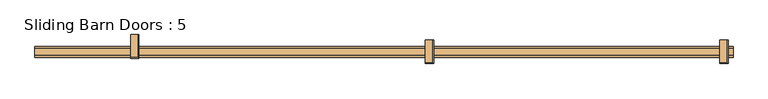
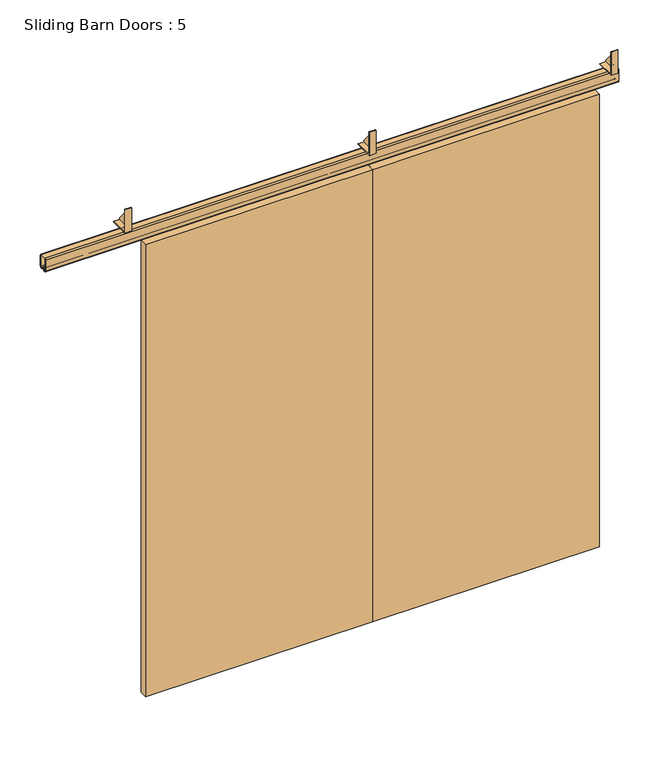
"""IFC4 building model written with IfcOpenShell, lengths in millimetres: door geometry, Sliding Barn Doors : 5."""

import ifcopenshell
import ifcopenshell.guid

model = None  # the IFC model being written
_history = None  # IfcOwnerHistory: only IFC2X3 demands one
_inside = {}  # id of a spatial element -> (the spatial element, [elements in it])
_under = {}  # id of a project, library or spatial element -> (it, [spatial elements below it])
_declared = {}  # id of a project -> (the project, [libraries it declares])
_typed = {}  # id of a type object -> (the type object, [elements of that type])
_made_of = {}  # id of a material, layer set ... -> (it, [elements and type objects made of it])


def new_model(schema):
    """Start an empty IFC model of exactly this schema.

    Asked for "IFC4X3", IfcOpenShell would pick the latest addendum, in which some entities
    have other attributes; the version numbers below select the first issue.
    IFC2X3 requires an IfcOwnerHistory on every rooted entity: one is made here for all.
    """
    global model, _history
    if schema == "IFC4X3":
        model = ifcopenshell.file(schema_version=(4, 3, 0, 0))
    else:
        model = ifcopenshell.file(schema=schema)
    _inside.clear()
    _under.clear()
    _declared.clear()
    _typed.clear()
    _made_of.clear()
    _history = None
    if model.schema == "IFC2X3":
        org = make("IfcOrganization", Name="unknown")
        user = make(
            "IfcPersonAndOrganization",
            ThePerson=make("IfcPerson", FamilyName="unknown"),
            TheOrganization=org,
        )
        app = make(
            "IfcApplication",
            ApplicationDeveloper=org,
            Version="unknown",
            ApplicationFullName="unknown",
            ApplicationIdentifier="unknown",
        )
        _history = make(
            "IfcOwnerHistory",
            OwningUser=user,
            OwningApplication=app,
            ChangeAction="ADDED",
            CreationDate=0,
        )
    return model


def make(cls, **values):
    """One entity of the class cls with the attributes given. An attribute that is None is left unset."""
    return model.create_entity(
        cls, **{name: value for name, value in values.items() if value is not None}
    )


def rooted(cls, **values):
    """An entity with a GlobalId (a new one), such as an element, a storey or a relation."""
    return make(cls, GlobalId=ifcopenshell.guid.new(), OwnerHistory=_history, **values)


def si_unit(unit_type, name, prefix=None):
    """IfcSIUnit, for example si_unit("LENGTHUNIT", "METRE", prefix="MILLI")."""
    return make("IfcSIUnit", UnitType=unit_type, Prefix=prefix, Name=name)


def assignment(units):
    """IfcUnitAssignment: the units of a project."""
    return None if units is None else make("IfcUnitAssignment", Units=units)


def point(xyz):
    """IfcCartesianPoint."""
    return None if xyz is None else make("IfcCartesianPoint", Coordinates=xyz)


def direction(xyz):
    """IfcDirection."""
    return None if xyz is None else make("IfcDirection", DirectionRatios=xyz)


def frame(location, z_axis=None, x_axis=None):
    """IfcAxis2Placement3D, a coordinate frame: its origin and axes. An axis left out is left unset."""
    return make(
        "IfcAxis2Placement3D",
        Location=point(location),
        Axis=direction(z_axis),
        RefDirection=direction(x_axis),
    )


def frame_2d(location, x_axis=None):
    """IfcAxis2Placement2D, a coordinate frame in the plane: its origin and x axis."""
    return make(
        "IfcAxis2Placement2D", Location=point(location), RefDirection=direction(x_axis)
    )


def origin():
    """The frame at (0, 0, 0) with its axes left unset."""
    return frame((0.0, 0.0, 0.0))


def place(relative_to, where):
    """IfcLocalPlacement: puts the frame where relative to a parent placement (None: the world)."""
    return make(
        "IfcLocalPlacement", PlacementRelTo=relative_to, RelativePlacement=where
    )


def context(
    kind, dimensions, precision=None, world=None, true_north=None, identifier=None
):
    """IfcGeometricRepresentationContext, for example the 3D "Model" context."""
    return make(
        "IfcGeometricRepresentationContext",
        ContextIdentifier=identifier,
        ContextType=kind,
        CoordinateSpaceDimension=dimensions,
        Precision=precision,
        WorldCoordinateSystem=world,
        TrueNorth=true_north,
    )


def project(units=None, contexts=None):
    """IfcProject with its units and contexts."""
    return rooted(
        "IfcProject",
        Name="project",
        RepresentationContexts=contexts,
        UnitsInContext=assignment(units),
    )


def spatial(cls, under=None, at=None, **own):
    """A site, building, storey or space (cls), placed at a placement, below another one or the project."""
    s = rooted(cls, ObjectPlacement=at, **own)
    if under is not None:
        _under.setdefault(under.id(), (under, []))[1].append(s)
    return s


def polyline(points):
    """IfcPolyline through the points."""
    return make("IfcPolyline", Points=[point(p) for p in points])


def circle_curve(where, radius):
    """IfcCircle in the frame where."""
    return make("IfcCircle", Position=where, Radius=radius)


def trimmed(basis, trim1, trim2, sense, master):
    """IfcTrimmedCurve: the piece of a basis curve between two trims."""
    return make(
        "IfcTrimmedCurve",
        BasisCurve=basis,
        Trim1=trim1,
        Trim2=trim2,
        SenseAgreement=sense,
        MasterRepresentation=master,
    )


def segment(curve, same_sense, transition):
    """IfcCompositeCurveSegment."""
    return make(
        "IfcCompositeCurveSegment",
        Transition=transition,
        SameSense=same_sense,
        ParentCurve=curve,
    )


def composite_curve(segments, self_intersect=None):
    """IfcCompositeCurve: segments joined end to end."""
    return make("IfcCompositeCurve", Segments=segments, SelfIntersect=self_intersect)


def outline(outer, holes=None, kind="AREA"):
    """IfcArbitraryClosedProfileDef: a profile drawn as a closed curve; with holes, ...WithVoids."""
    if holes is None:
        return make("IfcArbitraryClosedProfileDef", ProfileType=kind, OuterCurve=outer)
    return make(
        "IfcArbitraryProfileDefWithVoids",
        ProfileType=kind,
        OuterCurve=outer,
        InnerCurves=holes,
    )


def extrude(swept, where, along, depth):
    """IfcExtrudedAreaSolid: the profile swept, set in the frame where, extruded along a direction by depth."""
    return make(
        "IfcExtrudedAreaSolid",
        SweptArea=swept,
        Position=where,
        ExtrudedDirection=direction(along),
        Depth=depth,
    )


def shape(context_of_items, identifier, shape_type, items):
    """IfcShapeRepresentation: the items that make up one representation, for example the "Body"."""
    return make(
        "IfcShapeRepresentation",
        ContextOfItems=context_of_items,
        RepresentationIdentifier=identifier,
        RepresentationType=shape_type,
        Items=items,
    )


def source(mapping_origin, context_of_items, identifier, shape_type, items):
    """IfcRepresentationMap: a shape defined once, which mapped items show again and again."""
    return make(
        "IfcRepresentationMap",
        MappingOrigin=mapping_origin,
        MappedRepresentation=shape(context_of_items, identifier, shape_type, items),
    )


def transform(
    local_origin,
    x_axis=None,
    y_axis=None,
    z_axis=None,
    scale=None,
    scale2=None,
    scale3=None,
    uniform=True,
):
    """IfcCartesianTransformationOperator3D, or its non-uniform kind. x_axis, y_axis, z_axis: its Axis1, 2, 3."""
    if uniform:
        return make(
            "IfcCartesianTransformationOperator3D",
            Axis1=direction(x_axis),
            Axis2=direction(y_axis),
            LocalOrigin=point(local_origin),
            Scale=scale,
            Axis3=direction(z_axis),
        )
    return make(
        "IfcCartesianTransformationOperator3DnonUniform",
        Axis1=direction(x_axis),
        Axis2=direction(y_axis),
        LocalOrigin=point(local_origin),
        Scale=scale,
        Axis3=direction(z_axis),
        Scale2=scale2,
        Scale3=scale3,
    )


def mapped(mapping_source, mapping_target):
    """IfcMappedItem: shows the shape of a source again, moved by a transform."""
    return make(
        "IfcMappedItem", MappingSource=mapping_source, MappingTarget=mapping_target
    )


def made_of(thing, what):
    """Note that an element or type object is made of a material, layer set ...; save() writes the relation."""
    if what is not None:
        _made_of.setdefault(what.id(), (what, []))[1].append(thing)
    return thing


def element(
    cls,
    number,
    at=None,
    inside=None,
    cuts=None,
    type_object=None,
    material=None,
    context=None,
    identifier="Body",
    shape_type=None,
    held_by="IfcProductDefinitionShape",
    body=None,
    shapes=None,
    **own,
):
    """One element of the class cls, such as IfcWall. Its Tag is "e" and its number.

    at: its placement. inside: the storey or other place that contains it. cuts: it is an
    opening in that element (IfcRelVoidsElement). A single representation is given by context,
    identifier, shape_type and body (its items); several are given by shapes. held_by: the class
    of the entity that holds the representations. save() writes the other relations.
    """
    e = rooted(cls, Tag="e%d" % number, ObjectPlacement=at, **own)
    if body is not None:
        shapes = [shape(context, identifier, shape_type, body)]
    if shapes is not None:
        e.Representation = make(held_by, Representations=shapes)
    if inside is not None:
        _inside.setdefault(inside.id(), (inside, []))[1].append(e)
    if cuts is not None:
        rooted(
            "IfcRelVoidsElement", RelatingBuildingElement=cuts, RelatedOpeningElement=e
        )
    if type_object is not None:
        _typed.setdefault(type_object.id(), (type_object, []))[1].append(e)
    return made_of(e, material)


def aggregate(whole, parts):
    """IfcRelAggregates: a whole, such as a stair, and the parts it consists of."""
    return rooted("IfcRelAggregates", RelatingObject=whole, RelatedObjects=parts)


def save(model, path):
    """Write the relations noted so far, then the file.

    IfcRelAggregates (storeys below a building ...), IfcRelContainedInSpatialStructure (elements
    in a storey), IfcRelDefinesByType, IfcRelAssociatesMaterial and IfcRelDeclares: one each for
    every whole, place, type object, material and project.
    """
    for whole, parts in _under.values():
        aggregate(whole, parts)
    for where, things in _inside.values():
        rooted(
            "IfcRelContainedInSpatialStructure",
            RelatedElements=things,
            RelatingStructure=where,
        )
    for kind, things in _typed.values():
        rooted("IfcRelDefinesByType", RelatedObjects=things, RelatingType=kind)
    for what, things in _made_of.values():
        rooted("IfcRelAssociatesMaterial", RelatedObjects=things, RelatingMaterial=what)
    for by, libraries in _declared.values():
        rooted("IfcRelDeclares", RelatingContext=by, RelatedDefinitions=libraries)
    model.write(path)


def sliding_barn_doors_5_db2e6e72(model_context):
    return source(origin(), model_context, "Body", "SweptSolid", [
        extrude(outline(polyline([(158.75, 2152.65), (158.75, 2146.3), (79.375, 2146.3), (79.375, 2247.773), (158.75, 2152.65)])), frame((-1512.9371094, 0.0, 0.0), z_axis=(1.0, 0.0, 0.0), x_axis=(0.0, 1.0, 0.0)), (0.0, 0.0, 1.0), 3.175),
        extrude(outline(polyline([(76.2, 2143.125), (76.2, 2247.773), (79.375, 2247.773), (79.375, 2146.3), (158.75, 2146.3), (158.75, 2143.125), (76.2, 2143.125)])), frame((-1538.2378906, 0.0, 0.0), z_axis=(1.0, 0.0, 0.0), x_axis=(0.0, 1.0, 0.0)), (0.0, 0.0, 1.0), 28.4757812),
        extrude(outline(polyline([(139.7, 2152.65), (139.7, 2146.3), (60.325, 2146.3), (60.325, 2247.773), (139.7, 2152.65)])), frame((-484.2371094, 0.0, 0.0), z_axis=(1.0, 0.0, 0.0), x_axis=(0.0, 1.0, 0.0)), (0.0, 0.0, 1.0), 3.175),
        extrude(outline(polyline([(57.15, 2143.125), (57.15, 2247.773), (60.325, 2247.773), (60.325, 2146.3), (139.7, 2146.3), (139.7, 2143.125), (57.15, 2143.125)])), frame((-509.5378906, 0.0, 0.0), z_axis=(1.0, 0.0, 0.0), x_axis=(0.0, 1.0, 0.0)), (0.0, 0.0, 1.0), 28.4757813),
        extrude(outline(polyline([(139.7, 2152.65), (139.7, 2146.3), (60.325, 2146.3), (60.325, 2247.773), (139.7, 2152.65)])), frame((544.4628906, 0.0, 0.0), z_axis=(1.0, 0.0, 0.0), x_axis=(0.0, 1.0, 0.0)), (0.0, 0.0, 1.0), 3.175),
        extrude(outline(polyline([(57.15, 2143.125), (57.15, 2247.773), (60.325, 2247.773), (60.325, 2146.3), (139.7, 2146.3), (139.7, 2143.125), (57.15, 2143.125)])), frame((519.1621094, 0.0, 0.0), z_axis=(1.0, 0.0, 0.0), x_axis=(0.0, 1.0, 0.0)), (0.0, 0.0, 1.0), 28.4757813),
        extrude(outline(polyline([(-1346.454, 117.475), (-1295.146, 117.475), (-1295.146, 114.3), (-1346.454, 114.3), (-1346.454, 117.475)])), frame((0.0, 0.0, 1889.252), z_axis=(0.0, 0.0, 1.0), x_axis=(1.0, 0.0, 0.0)), (0.0, 0.0, 1.0), 168.148),
        extrude(outline(polyline([(-635.254, 117.475), (-583.946, 117.475), (-583.946, 114.3), (-635.254, 114.3), (-635.254, 117.475)])), frame((0.0, 0.0, 1889.252), z_axis=(0.0, 0.0, 1.0), x_axis=(1.0, 0.0, 0.0)), (0.0, 0.0, 1.0), 168.148),
        extrude(outline(polyline([(-381.254, 117.475), (-329.946, 117.475), (-329.946, 114.3), (-381.254, 114.3), (-381.254, 117.475)])), frame((0.0, 0.0, 1889.252), z_axis=(0.0, 0.0, 1.0), x_axis=(1.0, 0.0, 0.0)), (0.0, 0.0, 1.0), 168.148),
        extrude(outline(polyline([(329.946, 117.475), (381.254, 117.475), (381.254, 114.3), (329.946, 114.3), (329.946, 117.475)])), frame((0.0, 0.0, 1889.252), z_axis=(0.0, 0.0, 1.0), x_axis=(1.0, 0.0, 0.0)), (0.0, 0.0, 1.0), 168.148),
        extrude(outline(polyline([(-1447.8, 114.3), (-482.6, 114.3), (-482.6, 79.375), (-1447.8, 79.375), (-1447.8, 114.3)])), frame((0.0, 0.0, 25.4), z_axis=(0.0, 0.0, 1.0), x_axis=(1.0, 0.0, 0.0)), (0.0, 0.0, 1.0), 2032.0),
        extrude(outline(polyline([(-482.6, 114.3), (482.6, 114.3), (482.6, 79.375), (-482.6, 79.375), (-482.6, 114.3)])), frame((0.0, 0.0, 25.4), z_axis=(0.0, 0.0, 1.0), x_axis=(1.0, 0.0, 0.0)), (0.0, 0.0, 1.0), 2032.0),
        extrude(outline(composite_curve([segment(polyline([(85.725, 2143.125), (111.252, 2143.125)]), True, "CONTINUOUS"), segment(trimmed(circle_curve(frame_2d((111.252, 2136.775)), 6.35), [point((111.252, 2143.125))], [point((117.602, 2136.775))], False, "CARTESIAN"), True, "CONTINUOUS"), segment(polyline([(117.602, 2136.775), (117.602, 2088.515)]), True, "CONTINUOUS"), segment(trimmed(circle_curve(frame_2d((111.252, 2088.515)), 6.35), [point((117.602, 2088.515))], [point((111.252, 2082.165))], False, "CARTESIAN"), True, "CONTINUOUS"), segment(polyline([(111.252, 2082.165), (105.8433147, 2082.165)]), True, "CONTINUOUS"), segment(trimmed(circle_curve(frame_2d((105.8433147, 2083.7525)), 1.5875), [point((105.8433147, 2082.165))], [point((104.2849816, 2083.4495907))], False, "CARTESIAN"), True, "CONTINUOUS"), segment(polyline([(104.2849816, 2083.4495907), (102.8594659, 2090.7832331), (104.3756029, 2090.7832331), (105.7615251, 2083.6532812), (111.252, 2083.6532812)]), True, "CONTINUOUS"), segment(trimmed(circle_curve(frame_2d((111.252, 2088.515)), 4.8617187), [point((111.252, 2083.6532812))], [point((116.1137188, 2088.515))], True, "CARTESIAN"), True, "CONTINUOUS"), segment(polyline([(116.1137188, 2088.515), (116.1137188, 2136.775)]), True, "CONTINUOUS"), segment(trimmed(circle_curve(frame_2d((111.252, 2136.775)), 4.8617187), [point((116.1137188, 2136.775))], [point((111.252, 2141.6367187))], True, "CARTESIAN"), True, "CONTINUOUS"), segment(polyline([(111.252, 2141.6367187), (85.725, 2141.6367187)]), True, "CONTINUOUS"), segment(trimmed(circle_curve(frame_2d((85.725, 2136.775)), 4.8617187), [point((85.725, 2141.6367187))], [point((80.8632813, 2136.775))], True, "CARTESIAN"), True, "CONTINUOUS"), segment(polyline([(80.8632813, 2136.775), (80.8632813, 2088.515)]), True, "CONTINUOUS"), segment(trimmed(circle_curve(frame_2d((85.725, 2088.515)), 4.8617187), [point((80.8632813, 2088.515))], [point((85.725, 2083.6532812))], True, "CARTESIAN"), True, "CONTINUOUS"), segment(polyline([(85.725, 2083.6532812), (91.2154749, 2083.6532812), (92.6013971, 2090.7832331), (94.1175341, 2090.7832331), (92.6920184, 2083.4495907)]), True, "CONTINUOUS"), segment(trimmed(circle_curve(frame_2d((91.1336853, 2083.7525)), 1.5875), [point((92.6920184, 2083.4495907))], [point((91.1336853, 2082.165))], False, "CARTESIAN"), True, "CONTINUOUS"), segment(polyline([(91.1336853, 2082.165), (85.725, 2082.165)]), True, "CONTINUOUS"), segment(trimmed(circle_curve(frame_2d((85.725, 2088.515)), 6.35), [point((85.725, 2082.165))], [point((79.375, 2088.515))], False, "CARTESIAN"), True, "CONTINUOUS"), segment(polyline([(79.375, 2088.515), (79.375, 2136.775)]), True, "CONTINUOUS"), segment(trimmed(circle_curve(frame_2d((85.725, 2136.775)), 6.35), [point((79.375, 2136.775))], [point((85.725, 2143.125))], False, "CARTESIAN"), True, "CONTINUOUS")], self_intersect=False)), frame((-1873.25, 0.0, 0.0), z_axis=(1.0, 0.0, 0.0), x_axis=(0.0, 1.0, 0.0)), (0.0, 0.0, 1.0), 2438.4),
    ])


if __name__ == "__main__":
    model = new_model("IFC4")
    model_context = context("Model", 3, world=origin())
    ifc_project = project(units=[si_unit("LENGTHUNIT", "METRE", prefix="MILLI")], contexts=[model_context])
    site = spatial("IfcSite", under=ifc_project)
    building = spatial("IfcBuilding", under=site)
    placement = place(None, origin())
    sliding_barn_doors_5_shape = sliding_barn_doors_5_db2e6e72(model_context)
    element("IfcDoor", 1, ObjectType="Sliding Barn Doors : 5", at=placement, inside=building, context=model_context, shape_type="MappedRepresentation", body=[
        mapped(sliding_barn_doors_5_shape, transform((0.0, 0.0, 0.0), x_axis=(1.0, 0.0, 0.0), y_axis=(0.0, 1.0, 0.0), z_axis=(0.0, 0.0, 1.0))),
    ])
    save(model, "model.ifc")

# Revit data of these elements
# Type "Sliding Barn Doors : 5"
#   Type Mark = "46"
#   Analytic Construction = "<None>"
#   rail_overlap_left = 0' - 5 1/4"
#   rail_length = 8' - 0"
#   overlap_left = 0' - 2"
#   overlap = 0' - 0"
#   bracket_right = 3' - 7"
#   bracket_left = 0' - 4"
#   Thickness = 0' - 1 3/8"
#   Panel Width = 3' - 2"
#   Panel Height = 6' - 8"
#   Gap 2 = 0' - 0 1/2"
#   Gap 1 = 0' - 0 7/8"
#   Frame Projection Ext. = 0' - 1"
#   Frame Projection Int. = 0' - 1"
#   Frame Width = 0' - 3"
#   Height = 6' - 4"
#   Width = 2' - 10"
#   Bracket_offset = 0' - 5"
#   Door_4 = no
#   Door_3 = no
#   Hardware Material = Metal - Aluminum
#   Door Material = Closet_1
#   Function = (empty or 0)
#   Wall Closure = (empty or 0)
# Element 1 (IfcDoor, "Sliding Barn Doors : 5")
#   Materials on its faces: "Metal - Aluminum", "Closet_1"
# Materials
#   "Metal - Aluminum": class "Metal", colour RGB 247 247 247, transparency 0
#   "Closet_1": class "Paint", colour RGB 58 62 47, transparency 0, Cost = 0
